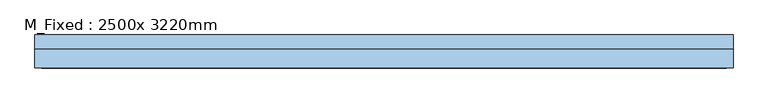
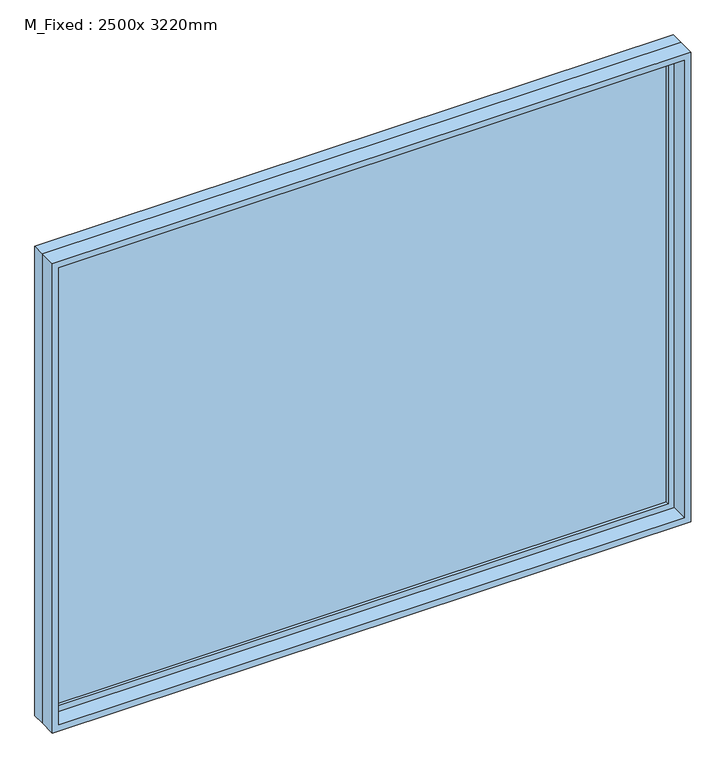
"""IFC4 building model written with IfcOpenShell, lengths in millimetres: window geometry, M_Fixed : 2500x 3220mm."""

from ifc_helpers import new_model, si_unit, frame, origin, place, context, project, spatial, polyline, outline, extrude, source, transform, mapped, element, save


def m_fixed_2500x_3220mm_df94f4d0(model_context):
    return source(origin(), model_context, "Body", "SweptSolid", [
        extrude(outline(polyline([(-1546.8, 54.2), (1546.8, 54.2), (1546.8, 42.2), (-1546.8, 42.2), (-1546.8, 54.2)])), frame((0.0, 0.0, 368.0), z_axis=(0.0, 0.0, 1.0), x_axis=(1.0, 0.0, 0.0)), (0.0, 0.0, 1.0), 2374.0),
        extrude(outline(polyline([(2786.0, -1590.8), (324.0, -1590.8), (324.0, 1590.8), (2786.0, 1590.8), (2786.0, -1590.8)]), holes=[polyline([(2742.0, -1546.8), (2742.0, 1546.8), (368.0, 1546.8), (368.0, -1546.8), (2742.0, -1546.8)])]), frame((0.0, 26.2, 0.0), z_axis=(0.0, 1.0, 0.0), x_axis=(0.0, 0.0, 1.0)), (0.0, 0.0, 1.0), 44.0),
        extrude(outline(polyline([(2805.0, -1609.8), (305.0, -1609.8), (305.0, 1609.8), (2805.0, 1609.8), (2805.0, -1609.8)]), holes=[polyline([(2786.0, -1590.8), (2786.0, 1590.8), (324.0, 1590.8), (324.0, -1590.8), (2786.0, -1590.8)])]), frame((0.0, 26.2, 0.0), z_axis=(0.0, 1.0, 0.0), x_axis=(0.0, 0.0, 1.0)), (0.0, 0.0, 1.0), 63.0),
        extrude(outline(polyline([(2805.0, -1609.8), (305.0, -1609.8), (305.0, 1609.8), (2805.0, 1609.8), (2805.0, -1609.8)]), holes=[polyline([(2773.0, -1577.8), (2773.0, 1577.8), (337.0, 1577.8), (337.0, -1577.8), (2773.0, -1577.8)])]), frame((0.0, -63.2, 0.0), z_axis=(0.0, 1.0, 0.0), x_axis=(0.0, 0.0, 1.0)), (0.0, 0.0, 1.0), 89.4),
    ])


if __name__ == "__main__":
    model = new_model("IFC4")
    model_context = context("Model", 3, world=origin())
    ifc_project = project(units=[si_unit("LENGTHUNIT", "METRE", prefix="MILLI")], contexts=[model_context])
    site = spatial("IfcSite", under=ifc_project)
    building = spatial("IfcBuilding", under=site)
    placement = place(None, origin())
    m_fixed_2500x_3220mm_shape = m_fixed_2500x_3220mm_df94f4d0(model_context)
    element("IfcWindow", 1, ObjectType="M_Fixed : 2500x 3220mm", at=placement, inside=building, context=model_context, shape_type="MappedRepresentation", body=[
        mapped(m_fixed_2500x_3220mm_shape, transform((0.0, 0.0, 0.0), x_axis=(1.0, 0.0, 0.0), y_axis=(0.0, 1.0, 0.0), z_axis=(0.0, 0.0, 1.0))),
    ])
    save(model, "model.ifc")

# Revit data of these elements
# Type "M_Fixed : 2500x 3220mm"
#   Type Mark = "26"
#   Height = 2500 mm
#   Default Sill Height = 305 mm
#   Width = 3219.6 mm
#   Window Inset = 19 mm
#   Frame Exterior Material = Sash
#   Frame Interior Material = Sash
#   Glass Pane Material = Glass
#   Sash = Sash
#   Wall Closure = (empty or 0)
# Element 1 (IfcWindow, "M_Fixed : 2500x 3220mm")
#   Materials on its faces: "Sash", "Glass"
# Materials
#   "Sash": class "Wood", colour RGB 136 99 55, transparency 0
#   "Glass": class "Glass", colour RGB 0 128 192, transparency 0.9, Description = "Soda Lime Glass", Cost = 0
